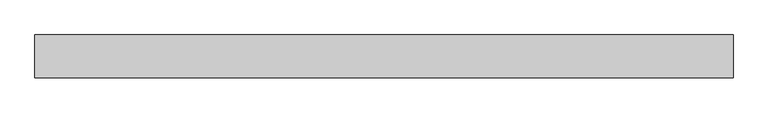
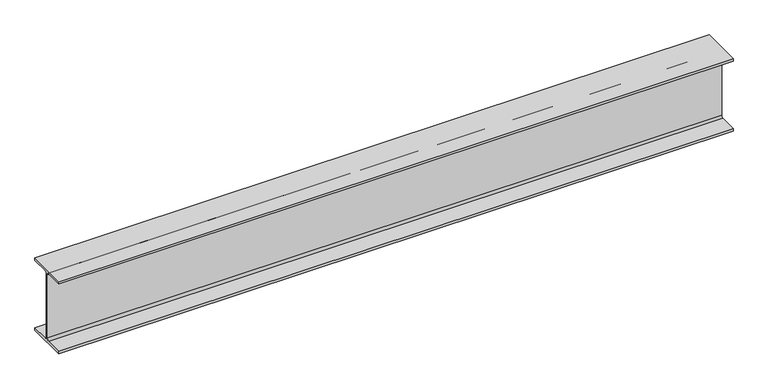
"""IFC4 building model written with IfcOpenShell, lengths in millimetres: beam geometry, Old_Steel Beam_H-KSD3502 : H_SB_ASB_H-250×125x6x9."""

from ifc_helpers import new_model, si_unit, point, frame, frame_2d, origin, place, context, project, spatial, polyline, circle_curve, trimmed, segment, composite_curve, outline, extrude, source, transform, mapped, element, save


def beam_4cb18809(model_context):
    return source(origin(), model_context, "Body", "SweptSolid", [
        extrude(outline(composite_curve([segment(polyline([(82.5, -141.5), (82.5, -151.7), (-82.5, -151.7), (-82.5, -141.5), (-11.9, -141.5)]), True, "CONTINUOUS"), segment(trimmed(circle_curve(frame_2d((-11.9, -132.6)), 8.9), [point((-11.9, -141.5))], [point((-3.0, -132.6))], True, "CARTESIAN"), True, "CONTINUOUS"), segment(polyline([(-3.0, -132.6), (-3.0, 132.6)]), True, "CONTINUOUS"), segment(trimmed(circle_curve(frame_2d((-11.9, 132.6)), 8.9), [point((-3.0, 132.6))], [point((-11.9, 141.5))], True, "CARTESIAN"), True, "CONTINUOUS"), segment(polyline([(-11.9, 141.5), (-82.5, 141.5), (-82.5, 151.7), (82.5, 151.7), (82.5, 141.5), (11.9, 141.5)]), True, "CONTINUOUS"), segment(trimmed(circle_curve(frame_2d((11.9, 132.6)), 8.9), [point((11.9, 141.5))], [point((3.0, 132.6))], True, "CARTESIAN"), True, "CONTINUOUS"), segment(polyline([(3.0, 132.6), (3.0, -132.6)]), True, "CONTINUOUS"), segment(trimmed(circle_curve(frame_2d((11.9, -132.6)), 8.9), [point((3.0, -132.6))], [point((11.9, -141.5))], True, "CARTESIAN"), True, "CONTINUOUS"), segment(polyline([(11.9, -141.5), (82.5, -141.5)]), True, "CONTINUOUS")], self_intersect=False)), frame((-1337.3, 0.0, 0.0), z_axis=(1.0, 0.0, 0.0), x_axis=(0.0, 1.0, 0.0)), (0.0, 0.0, 1.0), 2674.6),
    ])


if __name__ == "__main__":
    model = new_model("IFC4")
    model_context = context("Model", 3, world=origin())
    ifc_project = project(units=[si_unit("LENGTHUNIT", "METRE", prefix="MILLI")], contexts=[model_context])
    site = spatial("IfcSite", under=ifc_project)
    building = spatial("IfcBuilding", under=site)
    placement = place(None, origin())
    beam_shape = beam_4cb18809(model_context)
    element("IfcBeam", 1, ObjectType="Old_Steel Beam_H-KSD3502 : H_SB_ASB_H-250×125x6x9", at=placement, inside=building, context=model_context, shape_type="MappedRepresentation", body=[
        mapped(beam_shape, transform((0.0, 0.0, 0.0), x_axis=(1.0, 0.0, 0.0), y_axis=(0.0, 1.0, 0.0), z_axis=(0.0, 0.0, 1.0))),
    ])
    save(model, "model.ifc")

# Revit data of these elements
# Type "Old_Steel Beam_H-KSD3502 : H_SB_ASB_H-250×125x6x9"
#   Width = 12.5 cm
#   Web Thickness = 0.6 cm
#   Web Fillet = 1.2 cm
#   Warping Constant = 42539.8 cm⁶
#   Torsional Moment of Inertia = 7.8102 cm⁴
#   Torsional Modulus = 1.0 cm³
#   Section Area = 37.66 cm²
#   Plastic Modulus weak axis = 73.1 cm³
#   Plastic Modulus strong axis = 366.0 cm³
#   Perimeter = 0.97 m²/m
#   Nominal Weight = 29.60 kgf/m
#   Moment of Inertia weak axis = 294.00 cm⁴
#   Moment of Inertia strong axis = 4050.00 cm⁴
#   Height = 25.0 cm
#   Flange Thickness = 0.9 cm
#   Elastic Modulus weak axis = 47.0 cm³
#   Elastic Modulus strong axis = 324.0 cm³
#   Centroid Vertical = 12.5 cm
#   Centroid Horizontal = 6.25 cm
#   Length [instance default] = 1.5240 m
#   Structural Material [instance default] = Steel, 45-345
#   Assembly Code = ""
# Element 1 (IfcBeam, "Old_Steel Beam_H-KSD3502 : H_SB_ASB_H-250×125x6x9")
#   Structural Material = none
# Materials
#   "Steel, 45-345": class "Metal", colour RGB 189 187 185, transparency 0, Description = "Steel 345 MPa", Cost = 0
